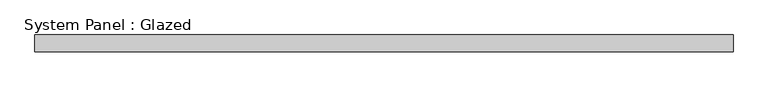
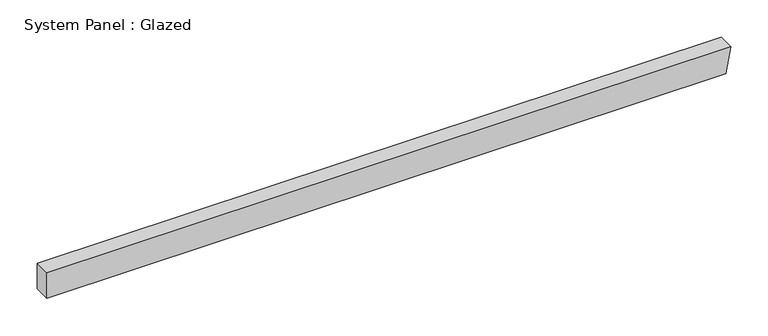
"""IFC4 building model written with IfcOpenShell, lengths in millimetres: plate geometry, System Panel : Glazed."""

from ifc_helpers import new_model, si_unit, frame, origin, place, context, project, spatial, polyline, outline, extrude, source, transform, mapped, element, save


def system_panel_glazed_3146f186(model_context):
    return source(origin(), model_context, "Body", "SweptSolid", [
        extrude(outline(polyline([(0.0, -529.1523878), (0.0, 521.789887), (41.9143134, 529.1523878), (41.9143134, -529.1523878), (0.0, -529.1523878)])), frame((0.0, -44.45, 0.0), z_axis=(0.0, 1.0, 0.0), x_axis=(0.0, 0.0, 1.0)), (0.0, 0.0, 1.0), 25.4),
    ])


if __name__ == "__main__":
    model = new_model("IFC4")
    model_context = context("Model", 3, world=origin())
    ifc_project = project(units=[si_unit("LENGTHUNIT", "METRE", prefix="MILLI")], contexts=[model_context])
    site = spatial("IfcSite", under=ifc_project)
    building = spatial("IfcBuilding", under=site)
    placement = place(None, origin())
    system_panel_glazed_shape = system_panel_glazed_3146f186(model_context)
    element("IfcPlate", 1, ObjectType="System Panel : Glazed", at=placement, inside=building, context=model_context, shape_type="MappedRepresentation", body=[
        mapped(system_panel_glazed_shape, transform((0.0, 0.0, 0.0), x_axis=(1.0, 0.0, 0.0), y_axis=(0.0, 1.0, 0.0), z_axis=(0.0, 0.0, 1.0))),
    ])
    save(model, "model.ifc")

# Revit data of these elements
# Type "System Panel : Glazed"
#   Construction Type Id = "GSP4R"
#   Analytic Construction = "1/8 in Pilkington single glazing"
#   Visual Light Transmittance = 0.9
#   Solar Heat Gain Coefficient = 0.86
#   Heat Transfer Coefficient (U) = 1.18115 BTU/(h·ft²·°F)
#   Define Thermal Properties by = 1
# Element 1 (IfcPlate, "System Panel : Glazed")
#   Materials on its faces: "Glass"
# Materials
#   "Glass": class "Glass", colour RGB 0 128 192, transparency 0.75, Description = "Soda Lime Glass", Cost = 0
